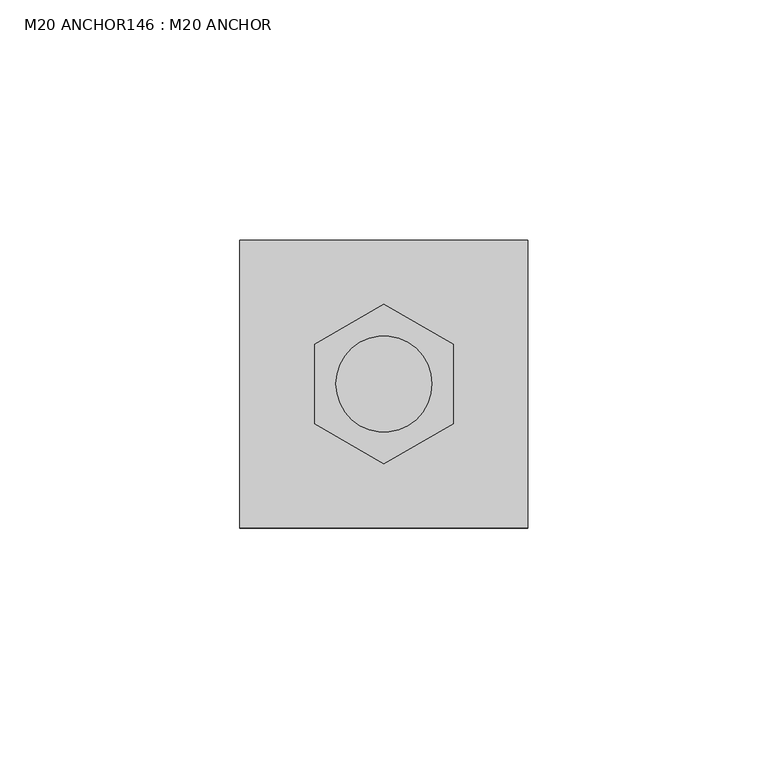
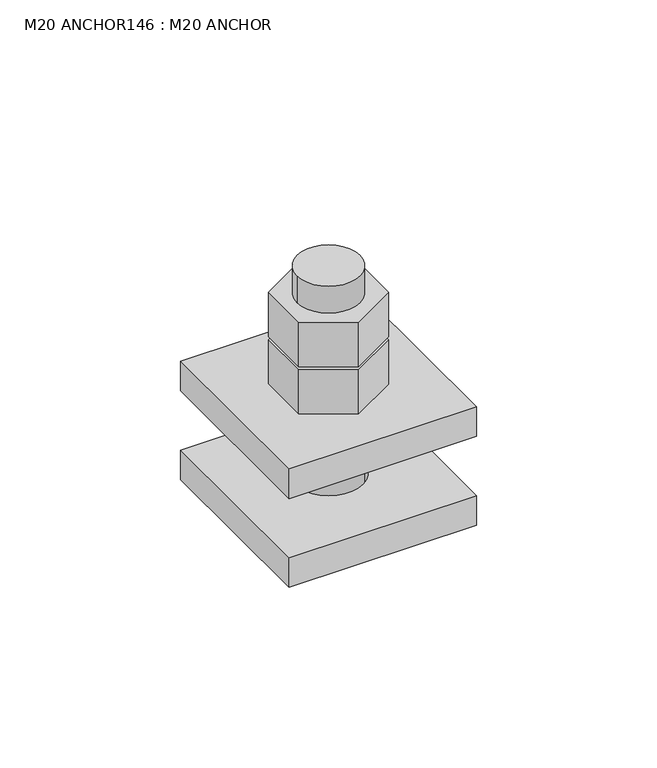
"""IFC4 building model written with IfcOpenShell, lengths in millimetres: fastener geometry, M20 ANCHOR146 : M20 ANCHOR."""

from ifc_helpers import new_model, si_unit, point, frame, frame_2d, origin, place, context, project, spatial, polyline, circle_curve, trimmed, segment, composite_curve, outline, extrude, source, transform, mapped, element, save


def m20_anchor146_m20_anchor_726ee2a0(model_context):
    return source(origin(), model_context, "Body", "SweptSolid", [
        extrude(outline(polyline([(5991.9144032, 22545.0952779), (5991.9144032, 22528.4582151), (5977.5062842, 22520.1396837), (5963.0981652, 22528.4582151), (5963.0981652, 22545.0952779), (5977.5062842, 22553.4138093), (5991.9144032, 22545.0952779)]), holes=[composite_curve([segment(trimmed(circle_curve(frame_2d((5977.5062842, 22536.7767465)), 10.0), [point((5967.5062842, 22536.7767465))], [point((5987.5062842, 22536.7767465))], True, "CARTESIAN"), True, "CONTINUOUS"), segment(trimmed(circle_curve(frame_2d((5977.5062842, 22536.7767465)), 10.0), [point((5987.5062842, 22536.7767465))], [point((5967.5062842, 22536.7767465))], True, "CARTESIAN"), True, "CONTINUOUS")], self_intersect=False)]), frame((0.0, 0.0, 246.0), z_axis=(0.0, 0.0, 1.0), x_axis=(1.0, 0.0, 0.0)), (0.0, 0.0, 1.0), 15.0),
        extrude(outline(polyline([(5991.9144032, 22545.0952779), (5991.9144032, 22528.4582151), (5977.5062842, 22520.1396837), (5963.0981652, 22528.4582151), (5963.0981652, 22545.0952779), (5977.5062842, 22553.4138093), (5991.9144032, 22545.0952779)]), holes=[composite_curve([segment(trimmed(circle_curve(frame_2d((5977.5062842, 22536.7767465)), 10.0), [point((5967.5062842, 22536.7767465))], [point((5987.5062842, 22536.7767465))], True, "CARTESIAN"), True, "CONTINUOUS"), segment(trimmed(circle_curve(frame_2d((5977.5062842, 22536.7767465)), 10.0), [point((5987.5062842, 22536.7767465))], [point((5967.5062842, 22536.7767465))], True, "CARTESIAN"), True, "CONTINUOUS")], self_intersect=False)]), frame((0.0, 0.0, 230.0), z_axis=(0.0, 0.0, 1.0), x_axis=(1.0, 0.0, 0.0)), (0.0, 0.0, 1.0), 15.0),
        extrude(outline(composite_curve([segment(trimmed(circle_curve(frame_2d((5977.5062842, 22536.7767465)), 10.0), [point((5967.5062842, 22536.7767465))], [point((5987.5062842, 22536.7767465))], False, "CARTESIAN"), True, "CONTINUOUS"), segment(trimmed(circle_curve(frame_2d((5977.5062842, 22536.7767465)), 10.0), [point((5987.5062842, 22536.7767465))], [point((5967.5062842, 22536.7767465))], False, "CARTESIAN"), True, "CONTINUOUS")], self_intersect=False)), frame((0.0, 0.0, 190.0), z_axis=(0.0, 0.0, 1.0), x_axis=(1.0, 0.0, 0.0)), (0.0, 0.0, 1.0), 80.0),
        extrude(outline(polyline([(6007.5062842, 22566.7767465), (6007.5062842, 22506.7767465), (5947.5062842, 22506.7767465), (5947.5062842, 22566.7767465), (6007.5062842, 22566.7767465)]), holes=[composite_curve([segment(trimmed(circle_curve(frame_2d((5977.5062842, 22536.7767465)), 11.0), [point((5966.5062842, 22536.7767465))], [point((5988.5062842, 22536.7767465))], True, "CARTESIAN"), True, "CONTINUOUS"), segment(trimmed(circle_curve(frame_2d((5977.5062842, 22536.7767465)), 11.0), [point((5988.5062842, 22536.7767465))], [point((5966.5062842, 22536.7767465))], True, "CARTESIAN"), True, "CONTINUOUS")], self_intersect=False)]), frame((0.0, 0.0, 190.0), z_axis=(0.0, 0.0, 1.0), x_axis=(1.0, 0.0, 0.0)), (0.0, 0.0, 1.0), 10.0),
        extrude(outline(polyline([(6007.5062842, 22566.7767465), (6007.5062842, 22506.7767465), (5947.5062842, 22506.7767465), (5947.5062842, 22566.7767465), (6007.5062842, 22566.7767465)]), holes=[composite_curve([segment(trimmed(circle_curve(frame_2d((5977.5062842, 22536.7767465)), 11.0), [point((5966.5062842, 22536.7767465))], [point((5988.5062842, 22536.7767465))], True, "CARTESIAN"), True, "CONTINUOUS"), segment(trimmed(circle_curve(frame_2d((5977.5062842, 22536.7767465)), 11.0), [point((5988.5062842, 22536.7767465))], [point((5966.5062842, 22536.7767465))], True, "CARTESIAN"), True, "CONTINUOUS")], self_intersect=False)]), frame((0.0, 0.0, 220.0), z_axis=(0.0, 0.0, 1.0), x_axis=(1.0, 0.0, 0.0)), (0.0, 0.0, 1.0), 10.0),
    ])


if __name__ == "__main__":
    model = new_model("IFC4")
    model_context = context("Model", 3, world=origin())
    ifc_project = project(units=[si_unit("LENGTHUNIT", "METRE", prefix="MILLI")], contexts=[model_context])
    site = spatial("IfcSite", under=ifc_project)
    building = spatial("IfcBuilding", under=site)
    placement = place(None, origin())
    m20_anchor146_m20_anchor_shape = m20_anchor146_m20_anchor_726ee2a0(model_context)
    element("IfcFastener", 1, ObjectType="M20 ANCHOR146 : M20 ANCHOR", at=placement, inside=building, context=model_context, shape_type="MappedRepresentation", body=[
        mapped(m20_anchor146_m20_anchor_shape, transform((0.0, 0.0, 0.0), x_axis=(1.0, 0.0, 0.0), y_axis=(0.0, 1.0, 0.0), z_axis=(0.0, 0.0, 1.0))),
    ])
    save(model, "model.ifc")
